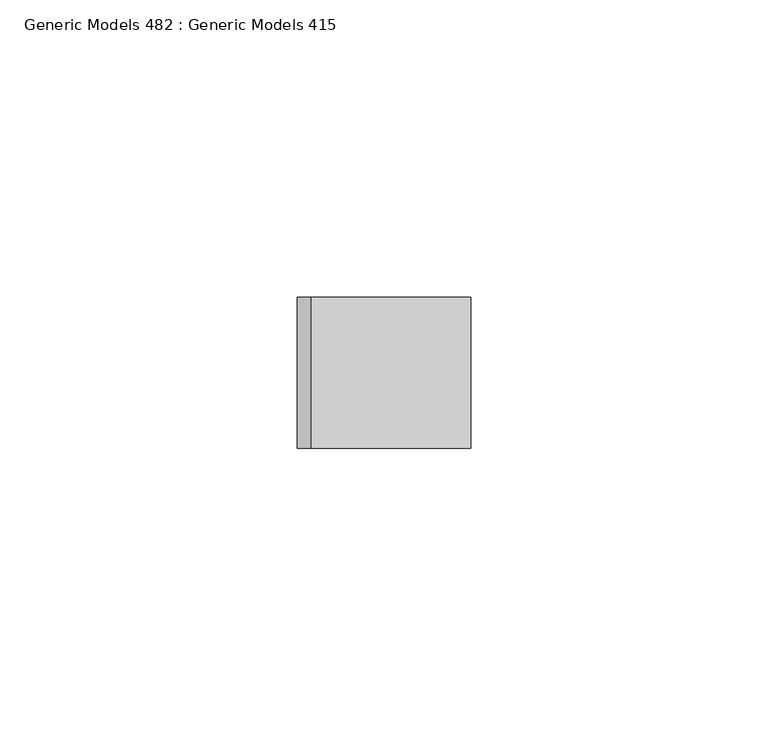
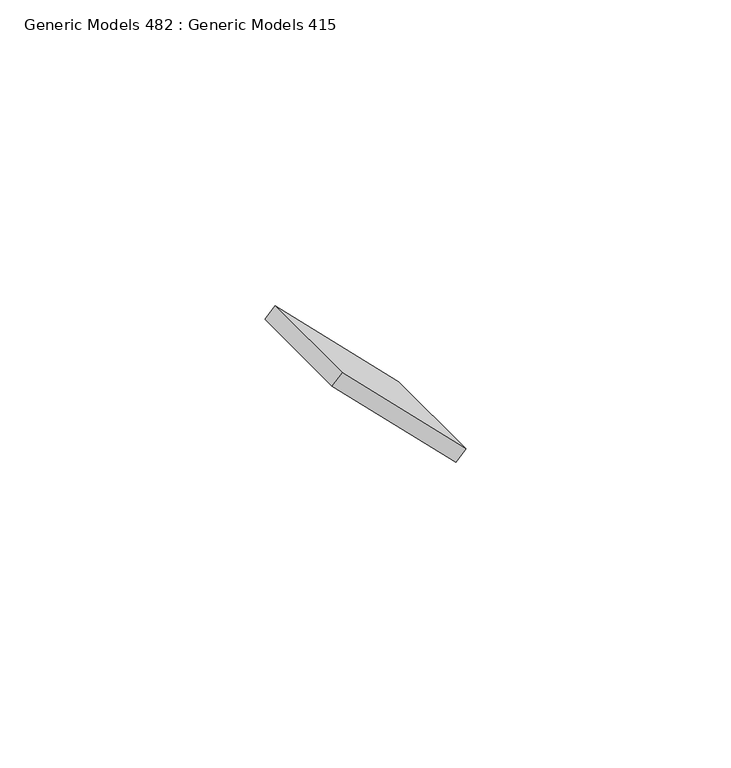
"""IFC4 building model written with IfcOpenShell, lengths in millimetres: proxy geometry, Generic Models 482 : Generic Models 415."""

from ifc_helpers import new_model, si_unit, frame, origin, place, context, project, spatial, polyline, outline, extrude, source, transform, mapped, element, save


def generic_models_482_generic_models_415_bb0f8a12(model_context):
    return source(origin(), model_context, "Body", "SweptSolid", [
        extrude(outline(polyline([(0.0, -38.1), (0.0, 0.0), (25.4, 0.0), (25.4, -38.1), (0.0, -38.1)])), frame((-6869.8996186, -4475.9863946, 127781.5002957), z_axis=(0.7071067811864907, 0.0, 0.7071067811866044), x_axis=(0.0, -1.0, 0.0)), (0.0, 0.0, 1.0), 3.175),
    ])


if __name__ == "__main__":
    model = new_model("IFC4")
    model_context = context("Model", 3, world=origin())
    ifc_project = project(units=[si_unit("LENGTHUNIT", "METRE", prefix="MILLI")], contexts=[model_context])
    site = spatial("IfcSite", under=ifc_project)
    building = spatial("IfcBuilding", under=site)
    placement = place(None, origin())
    generic_models_482_generic_models_415_shape = generic_models_482_generic_models_415_bb0f8a12(model_context)
    element("IfcBuildingElementProxy", 1, Name="Generic Models 482 : Generic Models 415", ObjectType="Generic Models 482 : Generic Models 415", at=placement, inside=building, context=model_context, shape_type="MappedRepresentation", body=[
        mapped(generic_models_482_generic_models_415_shape, transform((0.0, 0.0, 0.0), x_axis=(1.0, 0.0, 0.0), y_axis=(0.0, 1.0, 0.0), z_axis=(0.0, 0.0, 1.0))),
    ])
    save(model, "model.ifc")

# Revit data of these elements
# Element 1 (IfcBuildingElementProxy, "Generic Models 482 : Generic Models 415")
#   Materials on its faces: "_WELDED STEEL TABS FOR LOUVER ATTACHMENT"
# Materials
#   "_WELDED STEEL TABS FOR LOUVER ATTACHMENT": class "Metal", colour RGB 199 199 199, transparency 0, Description = "Structural steel 50ksi", Cost = 0
